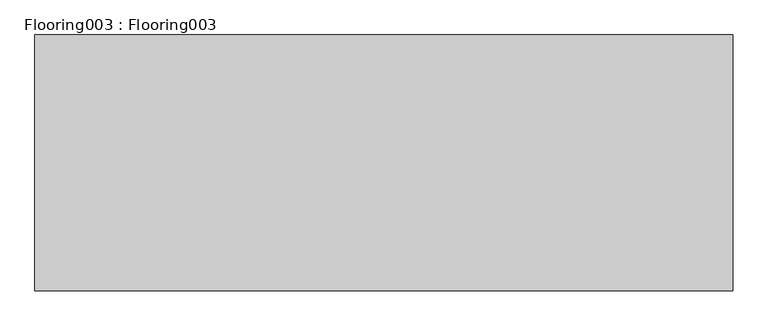
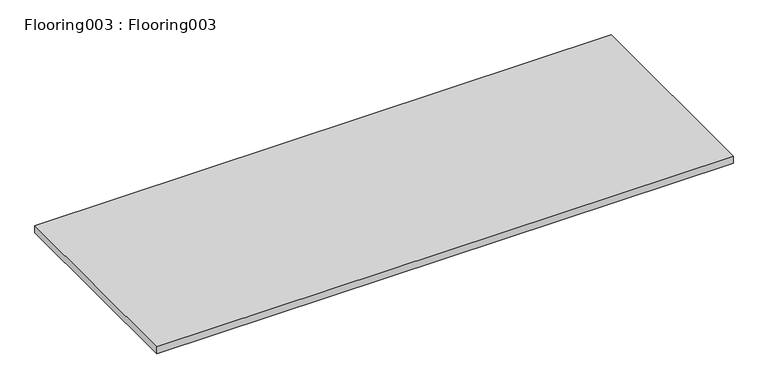
"""IFC4 building model written with IfcOpenShell, lengths in millimetres: proxy geometry, Flooring003 : Flooring003."""

from ifc_helpers import new_model, si_unit, frame, origin, place, context, project, spatial, polyline, outline, extrude, source, transform, mapped, element, save


def flooring003_flooring003_e13e8f99(model_context):
    return source(origin(), model_context, "Body", "SweptSolid", [
        extrude(outline(polyline([(14383.0178845, -3764.4167972), (14383.0178845, -4497.8417972), (12383.0178845, -4497.8417972), (12383.0178845, -3764.4167972), (14383.0178845, -3764.4167972)])), frame((0.0, 0.0, 36556.696), z_axis=(0.0, 0.0, 1.0), x_axis=(1.0, 0.0, 0.0)), (0.0, 0.0, 1.0), 25.4),
    ])


if __name__ == "__main__":
    model = new_model("IFC4")
    model_context = context("Model", 3, world=origin())
    ifc_project = project(units=[si_unit("LENGTHUNIT", "METRE", prefix="MILLI")], contexts=[model_context])
    site = spatial("IfcSite", under=ifc_project)
    building = spatial("IfcBuilding", under=site)
    placement = place(None, origin())
    flooring003_flooring003_shape = flooring003_flooring003_e13e8f99(model_context)
    element("IfcBuildingElementProxy", 1, Name="Flooring003 : Flooring003", ObjectType="Flooring003 : Flooring003", at=placement, inside=building, context=model_context, shape_type="MappedRepresentation", body=[
        mapped(flooring003_flooring003_shape, transform((0.0, 0.0, 0.0), x_axis=(1.0, 0.0, 0.0), y_axis=(0.0, 1.0, 0.0), z_axis=(0.0, 0.0, 1.0))),
    ])
    save(model, "model.ifc")

# Revit data of these elements
# Type "Flooring003 : Flooring003"
#   NameOverride = "Flooring003"
# Element 1 (IfcBuildingElementProxy, "Flooring003 : Flooring003")
#   Materials on its faces: "WOOD FLOORING (SPEC TBD)"
# Materials
#   "WOOD FLOORING (SPEC TBD)": class "Unassigned", colour RGB 201 162 125, transparency 0
